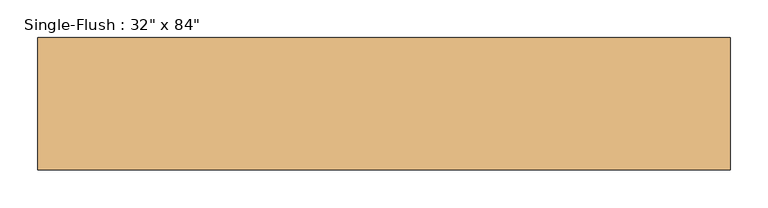
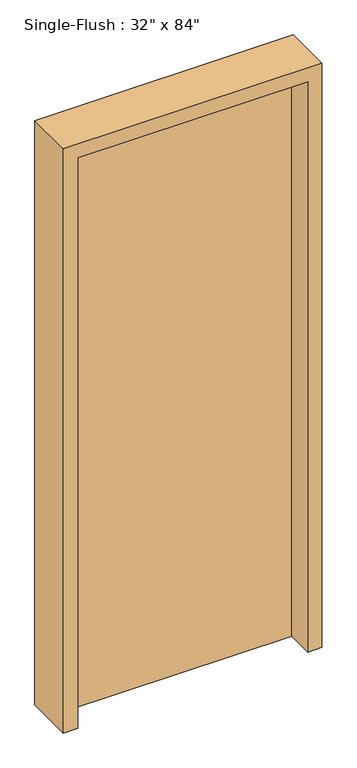
"""IFC4 building model written with IfcOpenShell, lengths in millimetres: door geometry."""

from ifc_helpers import new_model, si_unit, frame, origin, origin_with_axes, place, context, project, spatial, polyline, outline, extrude, source, transform, mapped, element, save


def door_dfb73b2b(model_context):
    return source(origin(), model_context, "Body", "SweptSolid", [
        extrude(outline(polyline([(2184.4, 457.2), (2184.4, -457.2), (0.0, -457.2), (0.0, -406.4), (2133.6, -406.4), (2133.6, 406.4), (0.0, 406.4), (0.0, 457.2), (2184.4, 457.2)])), frame((0.0, -87.3125, 0.0), z_axis=(0.0, 1.0, 0.0), x_axis=(0.0, 0.0, 1.0)), (0.0, 0.0, 1.0), 174.625),
        extrude(outline(polyline([(406.4, 11.1125), (-406.4, 11.1125), (-406.4, 61.9125), (406.4, 61.9125), (406.4, 11.1125)])), origin_with_axes(), (0.0, 0.0, 1.0), 2133.6),
    ])


if __name__ == "__main__":
    model = new_model("IFC4")
    model_context = context("Model", 3, world=origin())
    ifc_project = project(units=[si_unit("LENGTHUNIT", "METRE", prefix="MILLI")], contexts=[model_context])
    site = spatial("IfcSite", under=ifc_project)
    building = spatial("IfcBuilding", under=site)
    placement = place(None, origin())
    door_shape = door_dfb73b2b(model_context)
    element("IfcDoor", 1, ObjectType="Single-Flush : 32\" x 84\"", at=placement, inside=building, context=model_context, shape_type="MappedRepresentation", body=[
        mapped(door_shape, transform((0.0, 0.0, 0.0), x_axis=(1.0, 0.0, 0.0), y_axis=(0.0, 1.0, 0.0), z_axis=(0.0, 0.0, 1.0))),
    ])
    save(model, "model.ifc")

# Revit data of these elements
# Type "Single-Flush : 32\" x 84\""
#   Type Mark = "10"
#   Construction Type Id = "MDOOR"
#   Assembly Code = "C1020"
#   Analytic Construction = "Metal"
#   Thickness = 0' - 2"
#   Thermal Resistance (R) = 0.270117 (m²·K)/W
#   Heat Transfer Coefficient (U) = 3.7021 W/(m²·K)
#   Height = 7' - 0"
#   Trim Projection Ext = 0' - 1"
#   Trim Projection Int = 0' - 1"
#   Trim Width = 0' - 2"
#   Width = 2' - 8"
#   Door Material = Door - Panel
#   Frame Material = Door - Frame
#   Visual Light Transmittance = 0
#   Solar Heat Gain Coefficient = 0
#   Function = (empty or 0)
#   Wall Closure = (empty or 0)
# Element 1 (IfcDoor, "Single-Flush : 32\" x 84\"")
#   Materials on its faces: "Door - Frame", "Door - Panel"
# Materials
#   "Door - Panel": class "Wood", colour RGB 212 179 113, transparency 0, Cost = 0
#   "Door - Frame": class "Miscellaneous", colour RGB 65 65 65, transparency 0, Cost = 0
